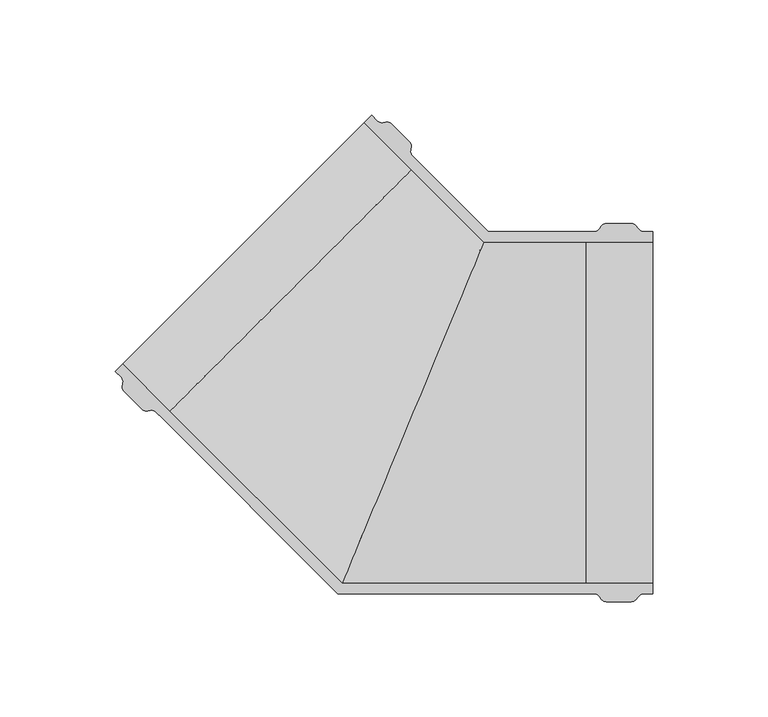
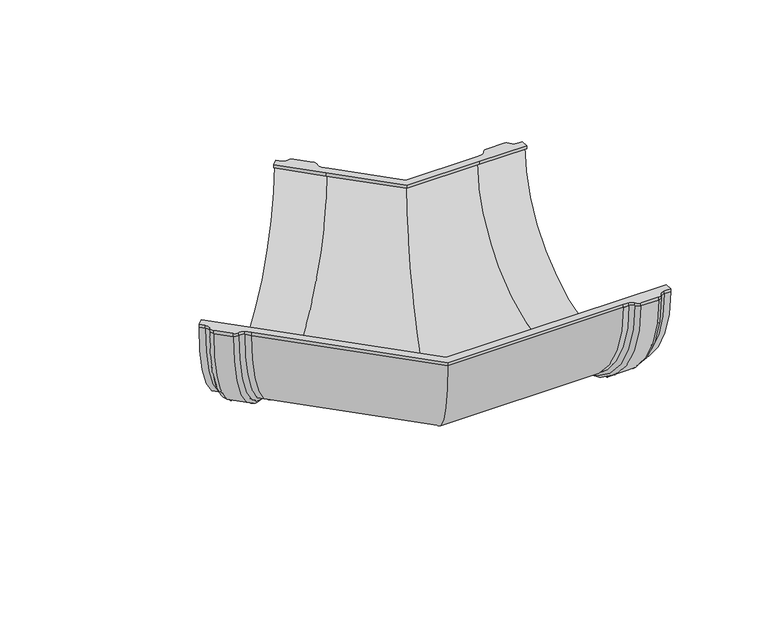
"""IFC4 building model written with IfcOpenShell, lengths in millimetres: proxy geometry, ↩ Угол универсальный 135 (слева) : ↩ Угол универсальный 135 (слева)."""

from ifc_helpers import new_model, si_unit, point, frame, origin, place, context, project, spatial, polyline, circle_curve, ellipse_curve, trimmed, source, transform, mapped, element, save
from ifc_brep_helpers import plane_surface, cylinder_surface, revolved_surface, advanced_brep


def generic_models_b2ec1c37(model_context):
    return source(origin(), model_context, "Body", "AdvancedBrep", [
        advanced_brep(
        [(-136.5214192, -78.5969124, 0.0), (-212.5505438, -2.5677877, 0.0), (-101.3820946, 108.6006614, 0.0), (-71.4004494, 78.6190162, 0.0), (-72.4445196, 76.0984077, 0.0), (-103.164434, 106.8183221, 0.0), (-210.7864614, -0.8037053, 0.0), (-135.4880436, -76.1021231, 0.0), (-28.9556587, 78.6190162, 0.0), (-28.9556587, -78.5969124, 0.0), (-28.9556587, -76.1021231, 0.0), (-28.9556587, 76.0984077, 0.0), (-233.0274697, 17.9047716, 0.0), (-233.0274697, 17.9047716, 2.0), (-229.8454892, 21.0867521, 2.0), (-229.8454892, 21.0867521, 0.0), (-231.2597028, 19.6725386, 0.0), (-123.6380507, 127.2941906, 0.0), (-125.0522642, 125.8799771, 0.0), (-125.0522642, 125.8799771, 2.0), (-121.8702837, 129.0619576, 2.0), (-121.8702837, 129.0619576, 0.0), (-119.4006442, 126.5923181, 0.0), (-230.5578302, 15.4351321, 0.0), (-116.2867573, 125.8825942, 0.0), (-229.8481063, 12.3212451, 0.0), (-113.1728703, 125.1728703, 0.0), (-229.1383824, 9.2073582, 0.0), (-105.5674711, 117.5674711, 0.0), (-221.5329832, 1.601959, 0.0), (-104.8577472, 114.4535841, 0.0), (-218.4190963, 0.8922351, 0.0), (-104.1480233, 111.3396972, 0.0), (-215.3052093, 0.1825112, 0.0), (-25.463061, -78.6, 0.0), (-25.463061, 78.6, 0.0), (-22.7593599, 80.3, 0.0), (-22.7593599, -80.3, 0.0), (-20.0556587, 82.0, 0.0), (-20.0556587, -82.0, 0.0), (-9.3, 82.0, 0.0), (-9.3, -82.0, 0.0), (-6.5962988, 80.3, 0.0), (-6.5962988, -80.3, 0.0), (-3.8925977, 78.6, 0.0), (-3.8925977, -78.6, 0.0), (0.0, 78.6, 0.0), (0.0, -78.6, 0.0), (0.0, 78.6, 2.0), (0.0, 74.1, 2.0), (0.0, 74.1, 0.0), (0.0, 76.1, 0.0), (0.0, -76.1, 0.0), (0.0, -74.1, 0.0), (0.0, -74.1, 2.0), (0.0, -78.6, 2.0), (-104.6088756, 105.4365885, 2.0), (-73.2722871, 74.1, 2.0), (-28.9556587, 74.1, 2.0), (-3.8925977, 78.6, 2.0), (-6.5962988, 80.3, 2.0), (-9.3, 82.0, 2.0), (-20.0556587, 82.0, 2.0), (-22.7593599, 80.3, 2.0), (-25.463061, 78.6, 2.0), (-28.9556587, 78.6, 2.0), (-71.4004494, 78.6190162, 2.0), (-101.3820946, 108.6006614, 2.0), (-104.1480233, 111.3396972, 2.0), (-104.8577472, 114.4535841, 2.0), (-105.5674711, 117.5674711, 2.0), (-113.1728703, 125.1728703, 2.0), (-116.2867573, 125.8825942, 2.0), (-119.4006442, 126.5923181, 2.0), (-136.5214192, -78.5969124, 2.0), (-28.9556587, -78.5969124, 2.0), (-25.463061, -78.6, 2.0), (-22.7593599, -80.3, 2.0), (-20.0556587, -82.0, 2.0), (-9.3, -82.0, 2.0), (-6.5962988, -80.3, 2.0), (-3.8925977, -78.6, 2.0), (-28.9556587, -74.1, 2.0), (-134.6596165, -74.1021231, 2.0), (-209.3722478, 0.6105082, 2.0), (-230.5578302, 15.4351321, 2.0), (-229.8481063, 12.3212451, 2.0), (-229.1383824, 9.2073582, 2.0), (-221.5329832, 1.601959, 2.0), (-218.4190963, 0.8922351, 2.0), (-215.3052093, 0.1825112, 2.0), (-212.5527271, -2.569971, 2.0), (-209.3707466, 0.6120095, 0.0), (-134.6596165, -74.1021231, 0.0), (-28.9556587, -74.1021231, 0.0), (-104.6088756, 105.4365885, 0.0), (-28.9556587, 74.1, 0.0), (-73.2722871, 74.1, 0.0)],
        [
            (0, 1),
            (1, 2, circle_curve(frame((-156.9663192, 53.0164368, 0.0), z_axis=(0.7071067811865459, -0.7071067811865492, 0.0), x_axis=(-0.7071067811865492, -0.7071067811865459, 0.0)), 78.6079643)),
            (2, 3),
            (3, 0, ellipse_curve(frame((-103.9609343, 0.0110519, 0.0), z_axis=(-0.9238795325112857, 0.38268343236509245, 0.0), x_axis=(0.38268343236509295, 0.9238795325112855, 0.0)), 85.0846474, 78.6079643)),
            (4, 5),
            (5, 6, circle_curve(frame((-156.9754477, 53.0073084, 0.0), z_axis=(-0.7071067811865459, 0.7071067811865492, 0.0), x_axis=(-0.7071067811865492, -0.7071067811865459, 0.0)), 76.1002654)),
            (6, 7),
            (7, 4, ellipse_curve(frame((-103.9662816, -0.0018577, 0.0), z_axis=(0.9238795325112857, -0.38268343236509245, 0.0), x_axis=(-0.38268343236509295, -0.9238795325112855, 0.0)), 82.3703337, 76.1002654)),
            (3, 8),
            (8, 9, circle_curve(frame((-28.9556587, 0.0110519, 0.0), z_axis=(-1.0, 0.0, 0.0), x_axis=(0.0, -1.0, 0.0)), 78.6079643)),
            (9, 0),
            (7, 10),
            (10, 11, circle_curve(frame((-28.9556587, -0.0018577, 0.0), z_axis=(1.0, 0.0, 0.0), x_axis=(0.0, -1.0, 0.0)), 76.1002654)),
            (11, 4),
            (12, 13),
            (13, 14),
            (14, 15),
            (15, 16),
            (16, 17, circle_curve(frame((-177.4488767, 73.4833646, 0.0), z_axis=(0.7071067811865475, -0.7071067811865477, 0.0), x_axis=(0.7071067811865477, 0.7071067811865475, 0.0)), 76.1)),
            (17, 18),
            (18, 19),
            (19, 20),
            (20, 21),
            (21, 12, circle_curve(frame((-177.4488767, 73.4833646, 0.0), z_axis=(-0.7071067811865475, 0.7071067811865477, 0.0), x_axis=(0.7071067811865477, 0.7071067811865475, 0.0)), 78.6)),
            (21, 22),
            (22, 23, circle_curve(frame((-174.9792372, 71.0137251, 0.0), z_axis=(-0.7071067811865475, 0.7071067811865477, 0.0), x_axis=(0.7071067811865477, 0.7071067811865475, 0.0)), 78.6)),
            (23, 12),
            (22, 24, circle_curve(frame((-117.2793239, 128.7136384, 0.0), z_axis=(0.0, 0.0, 1.0), x_axis=(0.7071067811865442, -0.7071067811865509, 0.0)), 3.0)),
            (24, 25, circle_curve(frame((-173.0674318, 69.1019197, 0.0), z_axis=(-0.7071067811865475, 0.7071067811865477, 0.0), x_axis=(0.7071067811865477, 0.7071067811865475, 0.0)), 80.3)),
            (25, 23, circle_curve(frame((-232.6791506, 13.3138118, 0.0), z_axis=(0.0, 0.0, 1.0), x_axis=(0.7071067811865507, -0.7071067811865445, 0.0)), 3.0)),
            (24, 26, circle_curve(frame((-115.2941906, 123.05155, 0.0), z_axis=(0.0, 0.0, -1.0), x_axis=(0.7071067811865442, -0.7071067811865509, 0.0)), 3.0)),
            (26, 27, circle_curve(frame((-171.1556264, 67.1901142, 0.0), z_axis=(-0.7071067811865475, 0.7071067811865477, 0.0), x_axis=(0.7071067811865477, 0.7071067811865475, 0.0)), 82.0)),
            (27, 25, circle_curve(frame((-227.0170621, 11.3286785, 0.0), z_axis=(0.0, 0.0, -1.0), x_axis=(0.7071067811865507, -0.7071067811865445, 0.0)), 3.0)),
            (26, 28),
            (28, 29, circle_curve(frame((-163.5502272, 59.584715, 0.0), z_axis=(-0.7071067811865475, 0.7071067811865477, 0.0), x_axis=(0.7071067811865477, 0.7071067811865475, 0.0)), 82.0)),
            (29, 27),
            (28, 30, circle_curve(frame((-107.6887914, 115.4461508, 0.0), z_axis=(0.0, 0.0, -1.0), x_axis=(-0.7071067811865442, 0.7071067811865509, 0.0)), 3.0)),
            (30, 31, circle_curve(frame((-161.6384217, 57.6729096, 0.0), z_axis=(-0.7071067811865475, 0.7071067811865477, 0.0), x_axis=(0.7071067811865477, 0.7071067811865475, 0.0)), 80.3)),
            (31, 29, circle_curve(frame((-219.4116629, 3.7232793, 0.0), z_axis=(0.0, 0.0, -1.0), x_axis=(-0.7071067811865507, 0.7071067811865445, 0.0)), 3.0)),
            (30, 32, circle_curve(frame((-102.0267029, 113.4610175, 0.0), z_axis=(0.0, 0.0, 1.0), x_axis=(-0.7071067811865442, 0.7071067811865509, 0.0)), 3.0)),
            (32, 33, circle_curve(frame((-159.7266163, 55.7611042, 0.0), z_axis=(-0.7071067811865475, 0.7071067811865477, 0.0), x_axis=(0.7071067811865477, 0.7071067811865475, 0.0)), 78.6)),
            (33, 31, circle_curve(frame((-217.4265296, -1.9388092, 0.0), z_axis=(0.0, 0.0, 1.0), x_axis=(-0.7071067811865507, 0.7071067811865445, 0.0)), 3.0)),
            (32, 2),
            (1, 33),
            (16, 6),
            (5, 17),
            (34, 9),
            (8, 35),
            (35, 34, circle_curve(frame((-25.463061, 0.0, 0.0), z_axis=(-1.0, 0.0, 0.0), x_axis=(0.0, 1.0, 0.0)), 78.6)),
            (35, 36, circle_curve(frame((-25.463061, 81.6, 0.0), z_axis=(0.0, 0.0, 1.0), x_axis=(1.0, 0.0, 0.0)), 3.0)),
            (36, 37, circle_curve(frame((-22.7593599, 0.0, 0.0), z_axis=(-1.0, 0.0, 0.0), x_axis=(0.0, 1.0, 0.0)), 80.3)),
            (37, 34, circle_curve(frame((-25.463061, -81.6, 0.0), z_axis=(0.0, 0.0, 1.0), x_axis=(1.0, 0.0, 0.0)), 3.0)),
            (36, 38, circle_curve(frame((-20.0556587, 79.0, 0.0), z_axis=(0.0, 0.0, -1.0), x_axis=(1.0, 0.0, 0.0)), 3.0)),
            (38, 39, circle_curve(frame((-20.0556587, 0.0, 0.0), z_axis=(-1.0, 0.0, 0.0), x_axis=(0.0, 1.0, 0.0)), 82.0)),
            (39, 37, circle_curve(frame((-20.0556587, -79.0, 0.0), z_axis=(0.0, 0.0, -1.0), x_axis=(1.0, 0.0, 0.0)), 3.0)),
            (38, 40),
            (40, 41, circle_curve(frame((-9.3, 0.0, 0.0), z_axis=(-1.0, 0.0, 0.0), x_axis=(0.0, 1.0, 0.0)), 82.0)),
            (41, 39),
            (40, 42, circle_curve(frame((-9.3, 79.0, 0.0), z_axis=(0.0, 0.0, -1.0), x_axis=(-1.0, 0.0, 0.0)), 3.0)),
            (42, 43, circle_curve(frame((-6.5962988, 0.0, 0.0), z_axis=(-1.0, 0.0, 0.0), x_axis=(0.0, 1.0, 0.0)), 80.3)),
            (43, 41, circle_curve(frame((-9.3, -79.0, 0.0), z_axis=(0.0, 0.0, -1.0), x_axis=(-1.0, 0.0, 0.0)), 3.0)),
            (42, 44, circle_curve(frame((-3.8925977, 81.6, 0.0), z_axis=(0.0, 0.0, 1.0), x_axis=(-1.0, 0.0, 0.0)), 3.0)),
            (44, 45, circle_curve(frame((-3.8925977, 0.0, 0.0), z_axis=(-1.0, 0.0, 0.0), x_axis=(0.0, 1.0, 0.0)), 78.6)),
            (45, 43, circle_curve(frame((-3.8925977, -81.6, 0.0), z_axis=(0.0, 0.0, 1.0), x_axis=(-1.0, 0.0, 0.0)), 3.0)),
            (44, 46),
            (46, 47, circle_curve(frame((0.0, 0.0, 0.0), z_axis=(-1.0, 0.0, 0.0), x_axis=(0.0, 1.0, 0.0)), 78.6)),
            (47, 45),
            (46, 48),
            (48, 49),
            (49, 50),
            (50, 51),
            (51, 52, circle_curve(frame((0.0, 0.0, 0.0), z_axis=(-1.0, 0.0, 0.0), x_axis=(0.0, 1.0, 0.0)), 76.1)),
            (52, 53),
            (53, 54),
            (54, 55),
            (55, 47),
            (51, 11),
            (10, 52),
            (56, 57),
            (57, 58),
            (58, 49),
            (48, 59),
            (59, 60, circle_curve(frame((-3.8925977, 81.6, 2.0), z_axis=(0.0, 0.0, -1.0), x_axis=(1.0, 0.0, 0.0)), 3.0)),
            (60, 61, circle_curve(frame((-9.3, 79.0, 2.0), z_axis=(0.0, 0.0, 1.0), x_axis=(1.0, 0.0, 0.0)), 3.0)),
            (61, 62),
            (62, 63, circle_curve(frame((-20.0556587, 79.0, 2.0), z_axis=(0.0, 0.0, 1.0), x_axis=(1.0, 0.0, 0.0)), 3.0)),
            (63, 64, circle_curve(frame((-25.463061, 81.6, 2.0), z_axis=(0.0, 0.0, -1.0), x_axis=(1.0, 0.0, 0.0)), 3.0)),
            (64, 65),
            (65, 66),
            (66, 67),
            (67, 68),
            (68, 69, circle_curve(frame((-102.0267029, 113.4610175, 2.0), z_axis=(0.0, 0.0, -1.0), x_axis=(1.0, 0.0, 0.0)), 3.0)),
            (69, 70, circle_curve(frame((-107.6887914, 115.4461508, 2.0), z_axis=(0.0, 0.0, 1.0), x_axis=(1.0, 0.0, 0.0)), 3.0)),
            (70, 71),
            (71, 72, circle_curve(frame((-115.2941906, 123.05155, 2.0), z_axis=(0.0, 0.0, 1.0), x_axis=(1.0, 0.0, 0.0)), 3.0)),
            (72, 73, circle_curve(frame((-117.2793239, 128.7136384, 2.0), z_axis=(0.0, 0.0, -1.0), x_axis=(1.0, 0.0, 0.0)), 3.0)),
            (73, 20),
            (19, 56),
            (74, 75),
            (75, 76),
            (76, 77, circle_curve(frame((-25.463061, -81.6, 2.0), z_axis=(0.0, 0.0, -1.0), x_axis=(1.0, 0.0, 0.0)), 3.0)),
            (77, 78, circle_curve(frame((-20.0556587, -79.0, 2.0), z_axis=(0.0, 0.0, 1.0), x_axis=(1.0, 0.0, 0.0)), 3.0)),
            (78, 79),
            (79, 80, circle_curve(frame((-9.3, -79.0, 2.0), z_axis=(0.0, 0.0, 1.0), x_axis=(1.0, 0.0, 0.0)), 3.0)),
            (80, 81, circle_curve(frame((-3.8925977, -81.6, 2.0), z_axis=(0.0, 0.0, -1.0), x_axis=(1.0, 0.0, 0.0)), 3.0)),
            (81, 55),
            (54, 82),
            (82, 83),
            (83, 84),
            (84, 14),
            (13, 85),
            (85, 86, circle_curve(frame((-232.6791506, 13.3138118, 2.0), z_axis=(0.0, 0.0, -1.0), x_axis=(1.0, 0.0, 0.0)), 3.0)),
            (86, 87, circle_curve(frame((-227.0170621, 11.3286785, 2.0), z_axis=(0.0, 0.0, 1.0), x_axis=(1.0, 0.0, 0.0)), 3.0)),
            (87, 88),
            (88, 89, circle_curve(frame((-219.4116629, 3.7232793, 2.0), z_axis=(0.0, 0.0, 1.0), x_axis=(1.0, 0.0, 0.0)), 3.0)),
            (89, 90, circle_curve(frame((-217.4265296, -1.9388092, 2.0), z_axis=(0.0, 0.0, -1.0), x_axis=(1.0, 0.0, 0.0)), 3.0)),
            (90, 91),
            (91, 74),
            (15, 92),
            (92, 93),
            (93, 94),
            (94, 53),
            (95, 18),
            (50, 96),
            (96, 97),
            (97, 95),
            (56, 95),
            (97, 57),
            (96, 58),
            (73, 22),
            (72, 24),
            (71, 26),
            (70, 28),
            (69, 30),
            (68, 32),
            (67, 2),
            (66, 3),
            (65, 8),
            (64, 35),
            (63, 36),
            (62, 38),
            (61, 40),
            (60, 42),
            (59, 44),
            (91, 1),
            (0, 74),
            (90, 33),
            (89, 31),
            (88, 29),
            (87, 27),
            (86, 25),
            (85, 23),
            (84, 92),
            (83, 93),
            (82, 94),
            (81, 45),
            (80, 43),
            (79, 41),
            (78, 39),
            (77, 37),
            (76, 34),
            (75, 9),
        ],
        [
            cylinder_surface(frame((-156.9663192, 53.0164368, 0.0), z_axis=(-0.7071067811865459, 0.7071067811865492, 0.0), x_axis=(-0.7071067811865492, -0.7071067811865459, 0.0)), 78.6079643),
            revolved_surface(polyline([(-135.48804361443615, -76.10212311443618, 0.0), (-210.78646141443625, -0.8037053144357309, 0.0)]), (-156.9754477, 53.0073084, 0.0), (0.7071067811865459, -0.7071067811865492, 0.0)),
            cylinder_surface(frame((-103.9655121, 0.0110519, 0.0), z_axis=(-1.0, 0.0, 0.0), x_axis=(0.0, -1.0, 0.0)), 78.6079643),
            revolved_surface(polyline([(-28.9556587, -76.1021231, 0.0), (-135.48804362537408, -76.1021231, 0.0)]), (-103.9655121, -0.0018577, 0.0), (1.0, 0.0, 0.0)),
            plane_surface(frame((-177.4488767, 73.4833646, 0.0), z_axis=(-0.7071067811865475, 0.7071067811865477, 0.0), x_axis=(0.7071067811865477, 0.7071067811865475, 0.0))),
            cylinder_surface(frame((-167.3529268, 63.3874146, 0.0), z_axis=(0.7071067811865475, -0.7071067811865477, 0.0), x_axis=(0.7071067811865477, 0.7071067811865475, 0.0)), 78.6),
            revolved_surface(trimmed(ellipse_curve(frame((-117.2793239, 128.7136384, 0.0), z_axis=(0.0, 0.0, 1.0), x_axis=(0.7071067811865442, -0.7071067811865509, 0.0)), 3.0, 3.0), [point((-119.4006442, 126.5923181, 0.0))], [point((-116.2867573, 125.8825942, 0.0))], True, "CARTESIAN"), (-167.3529268, 63.3874146, 0.0), (0.7071067811865475, -0.7071067811865477, 0.0)),
            revolved_surface(trimmed(ellipse_curve(frame((-115.2941906, 123.05155, 0.0), z_axis=(0.0, 0.0, -1.0), x_axis=(0.7071067811865442, -0.7071067811865509, 0.0)), 3.0, 3.0), [point((-116.2867573, 125.8825942, 0.0))], [point((-113.1728703, 125.1728703, 0.0))], True, "CARTESIAN"), (-167.3529268, 63.3874146, 0.0), (0.7071067811865475, -0.7071067811865477, 0.0)),
            cylinder_surface(frame((-167.3529268, 63.3874146, 0.0), z_axis=(0.7071067811865475, -0.7071067811865477, 0.0), x_axis=(0.7071067811865477, 0.7071067811865475, 0.0)), 82.0),
            revolved_surface(trimmed(ellipse_curve(frame((-107.6887914, 115.4461508, 0.0), z_axis=(0.0, 0.0, -1.0), x_axis=(-0.7071067811865442, 0.7071067811865509, 0.0)), 3.0, 3.0), [point((-105.5674711, 117.5674711, 0.0))], [point((-104.8577472, 114.4535841, 0.0))], True, "CARTESIAN"), (-167.3529268, 63.3874146, 0.0), (0.7071067811865475, -0.7071067811865477, 0.0)),
            revolved_surface(trimmed(ellipse_curve(frame((-102.0267029, 113.4610175, 0.0), z_axis=(0.0, 0.0, 1.0), x_axis=(-0.7071067811865442, 0.7071067811865509, 0.0)), 3.0, 3.0), [point((-104.8577472, 114.4535841, 0.0))], [point((-104.1480233, 111.3396972, 0.0))], True, "CARTESIAN"), (-167.3529268, 63.3874146, 0.0), (0.7071067811865475, -0.7071067811865477, 0.0)),
            revolved_surface(polyline([(-103.16330810170359, 106.81944799829613, 0.0), (-123.63805075170373, 127.29419064829627, 0.0)]), (-167.3529268, 63.3874146, 0.0), (0.7071067811865475, -0.7071067811865477, 0.0)),
            cylinder_surface(frame((-14.6778294, 0.0, 0.0), z_axis=(1.0, 0.0, 0.0), x_axis=(0.0, 1.0, 0.0)), 78.6),
            revolved_surface(trimmed(ellipse_curve(frame((-25.463061, 81.6, 0.0), z_axis=(0.0, 0.0, 1.0), x_axis=(1.0, 0.0, 0.0)), 3.0, 3.0), [point((-25.463061, 78.6, 0.0))], [point((-22.7593599, 80.3, 0.0))], True, "CARTESIAN"), (-14.6778294, 0.0, 0.0), (1.0, 0.0, 0.0)),
            revolved_surface(trimmed(ellipse_curve(frame((-20.0556587, 79.0, 0.0), z_axis=(0.0, 0.0, -1.0), x_axis=(1.0, 0.0, 0.0)), 3.0, 3.0), [point((-22.7593599, 80.3, 0.0))], [point((-20.0556587, 82.0, 0.0))], True, "CARTESIAN"), (-14.6778294, 0.0, 0.0), (1.0, 0.0, 0.0)),
            cylinder_surface(frame((-14.6778294, 0.0, 0.0), z_axis=(1.0, 0.0, 0.0), x_axis=(0.0, 1.0, 0.0)), 82.0),
            revolved_surface(trimmed(ellipse_curve(frame((-9.3, 79.0, 0.0), z_axis=(0.0, 0.0, -1.0), x_axis=(-1.0, 0.0, 0.0)), 3.0, 3.0), [point((-9.3, 82.0, 0.0))], [point((-6.5962988, 80.3, 0.0))], True, "CARTESIAN"), (-14.6778294, 0.0, 0.0), (1.0, 0.0, 0.0)),
            revolved_surface(trimmed(ellipse_curve(frame((-3.8925977, 81.6, 0.0), z_axis=(0.0, 0.0, 1.0), x_axis=(-1.0, 0.0, 0.0)), 3.0, 3.0), [point((-6.5962988, 80.3, 0.0))], [point((-3.8925977, 78.6, 0.0))], True, "CARTESIAN"), (-14.6778294, 0.0, 0.0), (1.0, 0.0, 0.0)),
            plane_surface(frame((0.0, 0.0, 0.0), z_axis=(1.0, 0.0, 0.0), x_axis=(0.0, 1.0, 0.0))),
            revolved_surface(polyline([(0.0, 76.1, 0.0), (-28.9556587, 76.1, 0.0)]), (-14.6778294, 0.0, 0.0), (1.0, 0.0, 0.0)),
            plane_surface(frame((-125.0836183, 125.9113311, 2.0), z_axis=(0.0, 0.0, 1.0), x_axis=(-0.7071067811865478, 0.7071067811865472, 0.0))),
            plane_surface(frame((-125.0836183, 125.9113311, 0.0), z_axis=(0.0, 0.0, -1.0), x_axis=(0.7071067811865478, -0.7071067811865472, 0.0))),
            plane_surface(frame((-73.2722871, 74.1, 2.0), z_axis=(-0.7071067811865492, -0.7071067811865459, 0.0), x_axis=(0.0, 0.0, -1.0))),
            plane_surface(frame((-28.9556587, 74.1, 2.0), z_axis=(0.0, -1.0, 0.0), x_axis=(0.0, 0.0, -1.0))),
            plane_surface(frame((0.0, 74.1, 2.0), z_axis=(0.0, -1.0, 0.0), x_axis=(0.0, 0.0, -1.0))),
            plane_surface(frame((-104.6088756, 105.4365885, 2.0), z_axis=(-0.7071067811865472, -0.7071067811865478, 0.0), x_axis=(0.0, 0.0, -1.0))),
            plane_surface(frame((-121.8702837, 129.0619576, 2.0), z_axis=(0.7071067811865402, 0.7071067811865548, 0.0), x_axis=(0.0, 0.0, -1.0))),
            revolved_surface(polyline([(-114.2793239, 128.7136384, 0.0), (-114.2793239, 128.7136384, 2.0)]), (-117.2793239, 128.7136384, 0.0), (0.0, 0.0, -1.0)),
            cylinder_surface(frame((-115.2941906, 123.05155, 0.0), z_axis=(0.0, 0.0, 1.0), x_axis=(1.0, 0.0, 0.0)), 3.0),
            plane_surface(frame((-113.1728703, 125.1728703, 2.0), z_axis=(0.7071067811865539, 0.7071067811865412, 0.0), x_axis=(0.0, 0.0, -1.0))),
            cylinder_surface(frame((-107.6887914, 115.4461508, 0.0), z_axis=(0.0, 0.0, 1.0), x_axis=(1.0, 0.0, 0.0)), 3.0),
            revolved_surface(polyline([(-99.0267029, 113.4610175, 0.0), (-99.0267029, 113.4610175, 2.0)]), (-102.0267029, 113.4610175, 0.0), (0.0, 0.0, -1.0)),
            plane_surface(frame((-104.1480233, 111.3396972, 2.0), z_axis=(0.7071067811865476, 0.7071067811865476, 0.0), x_axis=(0.0, 0.0, -1.0))),
            plane_surface(frame((-101.3820946, 108.6006614, 2.0), z_axis=(0.7071067811865489, 0.7071067811865461, 0.0), x_axis=(0.0, 0.0, -1.0))),
            plane_surface(frame((-71.4004494, 78.6190162, 2.0), z_axis=(0.0, 1.0, 0.0), x_axis=(0.0, 0.0, -1.0))),
            plane_surface(frame((-28.9556587, 78.6, 2.0), z_axis=(0.0, 1.0, 0.0), x_axis=(0.0, 0.0, -1.0))),
            revolved_surface(polyline([(-22.463061, 81.6, 0.0), (-22.463061, 81.6, 2.0)]), (-25.463061, 81.6, 0.0), (0.0, 0.0, -1.0)),
            cylinder_surface(frame((-20.0556587, 79.0, 0.0), z_axis=(0.0, 0.0, 1.0), x_axis=(1.0, 0.0, 0.0)), 3.0),
            plane_surface(frame((-20.0556587, 82.0, 2.0), z_axis=(0.0, 1.0, 0.0), x_axis=(0.0, 0.0, -1.0))),
            cylinder_surface(frame((-9.3, 79.0, 0.0), z_axis=(0.0, 0.0, 1.0), x_axis=(1.0, 0.0, 0.0)), 3.0),
            revolved_surface(polyline([(-0.8925977, 81.6, 0.0), (-0.8925977, 81.6, 2.0)]), (-3.8925977, 81.6, 0.0), (0.0, 0.0, -1.0)),
            plane_surface(frame((-3.8925977, 78.6, 2.0), z_axis=(0.0, 1.0, 0.0), x_axis=(0.0, 0.0, -1.0))),
            plane_surface(frame((-136.5214192, -78.5969124, 2.0), z_axis=(-0.7071067811865491, -0.707106781186546, 0.0), x_axis=(0.0, 0.0, -1.0))),
            plane_surface(frame((-212.5527271, -2.569971, 2.0), z_axis=(-0.7071067811865487, -0.7071067811865464, 0.0), x_axis=(0.0, 0.0, -1.0))),
            revolved_surface(polyline([(-214.4265296, -1.9388092, 0.0), (-214.4265296, -1.9388092, 2.0)]), (-217.4265296, -1.9388092, 0.0), (0.0, 0.0, -1.0)),
            cylinder_surface(frame((-219.4116629, 3.7232793, 0.0), z_axis=(0.0, 0.0, 1.0), x_axis=(1.0, 0.0, 0.0)), 3.0),
            plane_surface(frame((-221.5329832, 1.601959, 2.0), z_axis=(-0.7071067811865451, -0.70710678118655, 0.0), x_axis=(0.0, 0.0, -1.0))),
            cylinder_surface(frame((-227.0170621, 11.3286785, 0.0), z_axis=(0.0, 0.0, 1.0), x_axis=(1.0, 0.0, 0.0)), 3.0),
            revolved_surface(polyline([(-229.6791506, 13.3138118, 0.0), (-229.6791506, 13.3138118, 2.0)]), (-232.6791506, 13.3138118, 0.0), (0.0, 0.0, -1.0)),
            plane_surface(frame((-230.5578302, 15.4351321, 2.0), z_axis=(-0.7071067811865624, -0.7071067811865327, 0.0), x_axis=(0.0, 0.0, -1.0))),
            plane_surface(frame((-229.8454892, 21.0867521, 2.0), z_axis=(0.7071067811865476, 0.7071067811865476, 0.0), x_axis=(0.0, 0.0, -1.0))),
            plane_surface(frame((-209.3722478, 0.6105082, 2.0), z_axis=(0.7071067811865495, 0.7071067811865457, 0.0), x_axis=(0.0, 0.0, -1.0))),
            plane_surface(frame((-134.6596165, -74.1021231, 2.0), z_axis=(0.0, 1.0, 0.0), x_axis=(0.0, 0.0, -1.0))),
            plane_surface(frame((-28.9556587, -74.1, 2.0), z_axis=(0.0, 1.0, 0.0), x_axis=(0.0, 0.0, -1.0))),
            plane_surface(frame((0.0, -78.6, 2.0), z_axis=(0.0, -1.0, 0.0), x_axis=(0.0, 0.0, -1.0))),
            revolved_surface(polyline([(-0.8925977, -81.6, 0.0), (-0.8925977, -81.6, 2.0)]), (-3.8925977, -81.6, 0.0), (0.0, 0.0, -1.0)),
            cylinder_surface(frame((-9.3, -79.0, 0.0), z_axis=(0.0, 0.0, 1.0), x_axis=(1.0, 0.0, 0.0)), 3.0),
            plane_surface(frame((-9.3, -82.0, 2.0), z_axis=(0.0, -1.0, 0.0), x_axis=(0.0, 0.0, -1.0))),
            cylinder_surface(frame((-20.0556587, -79.0, 0.0), z_axis=(0.0, 0.0, 1.0), x_axis=(1.0, 0.0, 0.0)), 3.0),
            revolved_surface(polyline([(-22.463061, -81.6, 0.0), (-22.463061, -81.6, 2.0)]), (-25.463061, -81.6, 0.0), (0.0, 0.0, -1.0)),
            plane_surface(frame((-25.463061, -78.6, 2.0), z_axis=(0.0, -1.0, 0.0), x_axis=(0.0, 0.0, -1.0))),
            plane_surface(frame((-28.9556587, -78.5969124, 2.0), z_axis=(0.0, -1.0, 0.0), x_axis=(0.0, 0.0, -1.0))),
        ],
        [
            (0, [[1, 2, 3, 4]]),
            (1, [[5, 6, 7, 8]]),
            (2, [[9, 10, 11, -4]]),
            (3, [[12, 13, 14, -8]]),
            (4, [[15, 16, 17, 18, 19, 20, 21, 22, 23, 24]]),
            (5, [[25, 26, 27, -24]]),
            (6, [[28, 29, 30, -26]]),
            (7, [[31, 32, 33, -29]]),
            (8, [[34, 35, 36, -32]]),
            (9, [[37, 38, 39, -35]]),
            (10, [[40, 41, 42, -38]]),
            (5, [[43, -2, 44, -41]]),
            (11, [[45, -6, 46, -19]]),
            (12, [[47, -10, 48, 49]]),
            (13, [[50, 51, 52, -49]]),
            (14, [[53, 54, 55, -51]]),
            (15, [[56, 57, 58, -54]]),
            (16, [[59, 60, 61, -57]]),
            (17, [[62, 63, 64, -60]]),
            (12, [[65, 66, 67, -63]]),
            (18, [[68, 69, 70, 71, 72, 73, 74, 75, 76, -66]]),
            (19, [[77, -13, 78, -72]]),
            (20, [[79, 80, 81, -69, 82, 83, 84, 85, 86, 87, 88, 89, 90, 91, 92, 93, 94, 95, 96, 97, -22, 98]]),
            (20, [[99, 100, 101, 102, 103, 104, 105, 106, -75, 107, 108, 109, 110, -16, 111, 112, 113, 114, 115, 116, 117, 118]]),
            (21, [[-73, -78, -12, -7, -45, -18, 119, 120, 121, 122]]),
            (21, [[123, -20, -46, -5, -14, -77, -71, 124, 125, 126]]),
            (22, [[127, -126, 128, -79]]),
            (23, [[-128, -125, 129, -80]]),
            (24, [[-129, -124, -70, -81]]),
            (25, [[-21, -123, -127, -98]]),
            (26, [[130, -25, -23, -97]]),
            (27, [[131, -28, -130, -96]]),
            (28, [[132, -31, -131, -95]]),
            (29, [[133, -34, -132, -94]]),
            (30, [[134, -37, -133, -93]]),
            (31, [[135, -40, -134, -92]]),
            (32, [[136, -43, -135, -91]]),
            (33, [[137, -3, -136, -90]]),
            (34, [[138, -9, -137, -89]]),
            (35, [[139, -48, -138, -88]]),
            (36, [[140, -50, -139, -87]]),
            (37, [[141, -53, -140, -86]]),
            (38, [[142, -56, -141, -85]]),
            (39, [[143, -59, -142, -84]]),
            (40, [[144, -62, -143, -83]]),
            (41, [[-68, -65, -144, -82]]),
            (42, [[145, -1, 146, -118]]),
            (43, [[147, -44, -145, -117]]),
            (44, [[148, -42, -147, -116]]),
            (45, [[149, -39, -148, -115]]),
            (46, [[150, -36, -149, -114]]),
            (47, [[151, -33, -150, -113]]),
            (48, [[152, -30, -151, -112]]),
            (49, [[-15, -27, -152, -111]]),
            (50, [[153, -119, -17, -110]]),
            (51, [[154, -120, -153, -109]]),
            (52, [[155, -121, -154, -108]]),
            (53, [[-74, -122, -155, -107]]),
            (54, [[156, -67, -76, -106]]),
            (55, [[157, -64, -156, -105]]),
            (56, [[158, -61, -157, -104]]),
            (57, [[159, -58, -158, -103]]),
            (58, [[160, -55, -159, -102]]),
            (59, [[161, -52, -160, -101]]),
            (60, [[162, -47, -161, -100]]),
            (61, [[-146, -11, -162, -99]]),
        ],
    ),
    ])


if __name__ == "__main__":
    model = new_model("IFC4")
    model_context = context("Model", 3, world=origin())
    ifc_project = project(units=[si_unit("LENGTHUNIT", "METRE", prefix="MILLI")], contexts=[model_context])
    site = spatial("IfcSite", under=ifc_project)
    building = spatial("IfcBuilding", under=site)
    placement = place(None, origin())
    generic_models_shape = generic_models_b2ec1c37(model_context)
    element("IfcBuildingElementProxy", 1, Name="↩ Угол универсальный 135 (слева) : ↩ Угол универсальный 135 (слева)", ObjectType="↩ Угол универсальный 135 (слева) : ↩ Угол универсальный 135 (слева)", at=placement, inside=building, context=model_context, shape_type="MappedRepresentation", body=[
        mapped(generic_models_shape, transform((0.0, 0.0, 0.0), x_axis=(1.0, 0.0, 0.0), y_axis=(0.0, 1.0, 0.0), z_axis=(0.0, 0.0, 1.0))),
    ])
    save(model, "model.ifc")

# Revit data of these elements
# Type "↩ Угол универсальный 135 (слева) : ↩ Угол универсальный 135 (слева)"
#   Description = "Используется для изменения направления потока воды, монтируется на внешних и внутренних углах кровли."
#   Manufacturer = "ТехноНИКОЛЬ"
#   Model = "Комплектующие к водосточным системам"
#   URL = "https://tn-vodostok.ru/catalog/pvh/"
#   ADSK_Обозначение = "ТехноНИКОЛЬ"
#   ADSK_Наименование краткое = "Угол 135°"
#   ADSK_Наименование = "Угол универсальный 135°"
#   ADSK_Масса_Текст = ""
#   ADSK_Марка = ""
#   ADSK_Код изделия = ""
#   ADSK_Завод-изготовитель = "ТехноНИКОЛЬ"
#   ADSK_Единица измерения = "шт."
#   ADSK_Группирование = "Комплектующие к водосточным системам"
#   ADSK_URL страницы изделия = "https://tn-vodostok.ru/catalog/pvh/"
#   ADSK_URL документации изделия = "https://tn-vodostok.ru/upload/iblock/c42/c427963cb77eb5c3c51f0cfb870e9e52.pdf"
#   Угол поворота кронштейна [instance default] = 0.00°
#   Длина пластины [instance default] = 0 mm
#   ADSK_Размер_Ширина = 164 mm
#   ADSK_Размер_Высота = 82 mm
#   ADSK_Количество = 1
#   Видимость_Защитная решетка [instance default] = yes
#   Материал_Защитная решетка [instance default] = none
#   ADSK_Материал [instance default] = TN_Пластик_Коричневый_RAL8019
#   Default Elevation = 0
# Element 1 (IfcBuildingElementProxy, "↩ Угол универсальный 135 (слева) : ↩ Угол универсальный 135 (слева)")
#   Угол поворота кронштейна = 45.00°
#   Длина пластины = 200 mm
#   Видимость_Защитная решетка = no
#   Материал_Защитная решетка = TN_Пластик_Решетка_Коричневый_RAL8019
#   Materials on its faces: "TN_Пластик_Коричневый_RAL8019"
# Materials
#   "TN_Пластик_Коричневый_RAL8019": class "Типовые", colour RGB 61 54 53, transparency 0, Cost = 0
#   "TN_Пластик_Решетка_Коричневый_RAL8019": class "Типовые", colour RGB 61 54 53, transparency 0.25, Cost = 0
